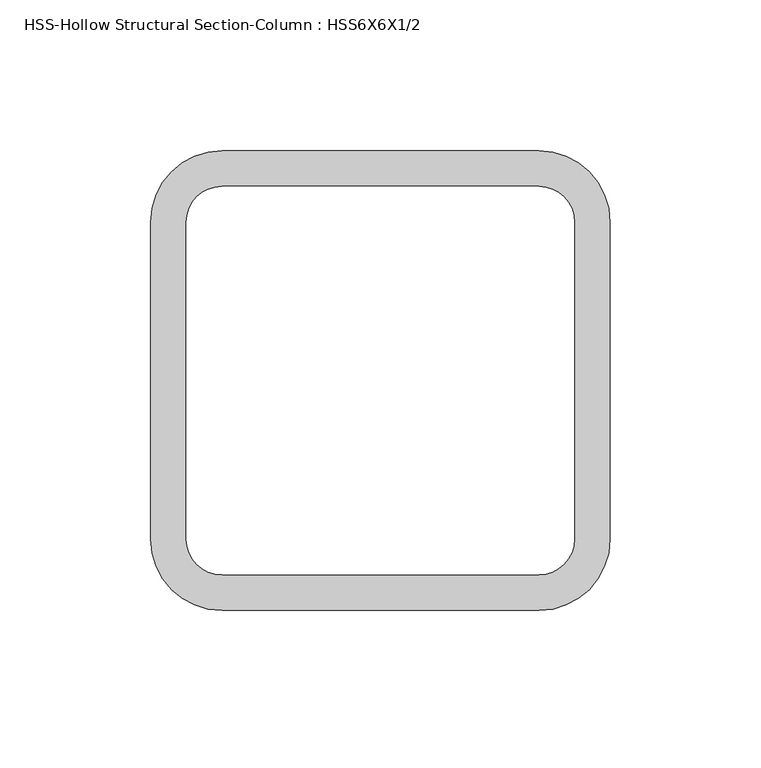
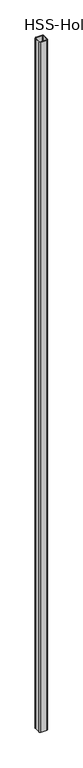
"""IFC4 building model written with IfcOpenShell, lengths in millimetres: column geometry, HSS-Hollow Structural Section-Column : HSS6X6X1/2."""

import ifcopenshell
import ifcopenshell.guid

model = None  # the IFC model being written
_history = None  # IfcOwnerHistory: only IFC2X3 demands one
_inside = {}  # id of a spatial element -> (the spatial element, [elements in it])
_under = {}  # id of a project, library or spatial element -> (it, [spatial elements below it])
_declared = {}  # id of a project -> (the project, [libraries it declares])
_typed = {}  # id of a type object -> (the type object, [elements of that type])
_made_of = {}  # id of a material, layer set ... -> (it, [elements and type objects made of it])


def new_model(schema):
    """Start an empty IFC model of exactly this schema.

    Asked for "IFC4X3", IfcOpenShell would pick the latest addendum, in which some entities
    have other attributes; the version numbers below select the first issue.
    IFC2X3 requires an IfcOwnerHistory on every rooted entity: one is made here for all.
    """
    global model, _history
    if schema == "IFC4X3":
        model = ifcopenshell.file(schema_version=(4, 3, 0, 0))
    else:
        model = ifcopenshell.file(schema=schema)
    _inside.clear()
    _under.clear()
    _declared.clear()
    _typed.clear()
    _made_of.clear()
    _history = None
    if model.schema == "IFC2X3":
        org = make("IfcOrganization", Name="unknown")
        user = make(
            "IfcPersonAndOrganization",
            ThePerson=make("IfcPerson", FamilyName="unknown"),
            TheOrganization=org,
        )
        app = make(
            "IfcApplication",
            ApplicationDeveloper=org,
            Version="unknown",
            ApplicationFullName="unknown",
            ApplicationIdentifier="unknown",
        )
        _history = make(
            "IfcOwnerHistory",
            OwningUser=user,
            OwningApplication=app,
            ChangeAction="ADDED",
            CreationDate=0,
        )
    return model


def make(cls, **values):
    """One entity of the class cls with the attributes given. An attribute that is None is left unset."""
    return model.create_entity(
        cls, **{name: value for name, value in values.items() if value is not None}
    )


def rooted(cls, **values):
    """An entity with a GlobalId (a new one), such as an element, a storey or a relation."""
    return make(cls, GlobalId=ifcopenshell.guid.new(), OwnerHistory=_history, **values)


def si_unit(unit_type, name, prefix=None):
    """IfcSIUnit, for example si_unit("LENGTHUNIT", "METRE", prefix="MILLI")."""
    return make("IfcSIUnit", UnitType=unit_type, Prefix=prefix, Name=name)


def assignment(units):
    """IfcUnitAssignment: the units of a project."""
    return None if units is None else make("IfcUnitAssignment", Units=units)


def point(xyz):
    """IfcCartesianPoint."""
    return None if xyz is None else make("IfcCartesianPoint", Coordinates=xyz)


def direction(xyz):
    """IfcDirection."""
    return None if xyz is None else make("IfcDirection", DirectionRatios=xyz)


def frame(location, z_axis=None, x_axis=None):
    """IfcAxis2Placement3D, a coordinate frame: its origin and axes. An axis left out is left unset."""
    return make(
        "IfcAxis2Placement3D",
        Location=point(location),
        Axis=direction(z_axis),
        RefDirection=direction(x_axis),
    )


def frame_2d(location, x_axis=None):
    """IfcAxis2Placement2D, a coordinate frame in the plane: its origin and x axis."""
    return make(
        "IfcAxis2Placement2D", Location=point(location), RefDirection=direction(x_axis)
    )


def origin():
    """The frame at (0, 0, 0) with its axes left unset."""
    return frame((0.0, 0.0, 0.0))


def place(relative_to, where):
    """IfcLocalPlacement: puts the frame where relative to a parent placement (None: the world)."""
    return make(
        "IfcLocalPlacement", PlacementRelTo=relative_to, RelativePlacement=where
    )


def context(
    kind, dimensions, precision=None, world=None, true_north=None, identifier=None
):
    """IfcGeometricRepresentationContext, for example the 3D "Model" context."""
    return make(
        "IfcGeometricRepresentationContext",
        ContextIdentifier=identifier,
        ContextType=kind,
        CoordinateSpaceDimension=dimensions,
        Precision=precision,
        WorldCoordinateSystem=world,
        TrueNorth=true_north,
    )


def project(units=None, contexts=None):
    """IfcProject with its units and contexts."""
    return rooted(
        "IfcProject",
        Name="project",
        RepresentationContexts=contexts,
        UnitsInContext=assignment(units),
    )


def spatial(cls, under=None, at=None, **own):
    """A site, building, storey or space (cls), placed at a placement, below another one or the project."""
    s = rooted(cls, ObjectPlacement=at, **own)
    if under is not None:
        _under.setdefault(under.id(), (under, []))[1].append(s)
    return s


def polyline(points):
    """IfcPolyline through the points."""
    return make("IfcPolyline", Points=[point(p) for p in points])


def circle_curve(where, radius):
    """IfcCircle in the frame where."""
    return make("IfcCircle", Position=where, Radius=radius)


def trimmed(basis, trim1, trim2, sense, master):
    """IfcTrimmedCurve: the piece of a basis curve between two trims."""
    return make(
        "IfcTrimmedCurve",
        BasisCurve=basis,
        Trim1=trim1,
        Trim2=trim2,
        SenseAgreement=sense,
        MasterRepresentation=master,
    )


def segment(curve, same_sense, transition):
    """IfcCompositeCurveSegment."""
    return make(
        "IfcCompositeCurveSegment",
        Transition=transition,
        SameSense=same_sense,
        ParentCurve=curve,
    )


def composite_curve(segments, self_intersect=None):
    """IfcCompositeCurve: segments joined end to end."""
    return make("IfcCompositeCurve", Segments=segments, SelfIntersect=self_intersect)


def outline(outer, holes=None, kind="AREA"):
    """IfcArbitraryClosedProfileDef: a profile drawn as a closed curve; with holes, ...WithVoids."""
    if holes is None:
        return make("IfcArbitraryClosedProfileDef", ProfileType=kind, OuterCurve=outer)
    return make(
        "IfcArbitraryProfileDefWithVoids",
        ProfileType=kind,
        OuterCurve=outer,
        InnerCurves=holes,
    )


def extrude(swept, where, along, depth):
    """IfcExtrudedAreaSolid: the profile swept, set in the frame where, extruded along a direction by depth."""
    return make(
        "IfcExtrudedAreaSolid",
        SweptArea=swept,
        Position=where,
        ExtrudedDirection=direction(along),
        Depth=depth,
    )


def shape(context_of_items, identifier, shape_type, items):
    """IfcShapeRepresentation: the items that make up one representation, for example the "Body"."""
    return make(
        "IfcShapeRepresentation",
        ContextOfItems=context_of_items,
        RepresentationIdentifier=identifier,
        RepresentationType=shape_type,
        Items=items,
    )


def source(mapping_origin, context_of_items, identifier, shape_type, items):
    """IfcRepresentationMap: a shape defined once, which mapped items show again and again."""
    return make(
        "IfcRepresentationMap",
        MappingOrigin=mapping_origin,
        MappedRepresentation=shape(context_of_items, identifier, shape_type, items),
    )


def transform(
    local_origin,
    x_axis=None,
    y_axis=None,
    z_axis=None,
    scale=None,
    scale2=None,
    scale3=None,
    uniform=True,
):
    """IfcCartesianTransformationOperator3D, or its non-uniform kind. x_axis, y_axis, z_axis: its Axis1, 2, 3."""
    if uniform:
        return make(
            "IfcCartesianTransformationOperator3D",
            Axis1=direction(x_axis),
            Axis2=direction(y_axis),
            LocalOrigin=point(local_origin),
            Scale=scale,
            Axis3=direction(z_axis),
        )
    return make(
        "IfcCartesianTransformationOperator3DnonUniform",
        Axis1=direction(x_axis),
        Axis2=direction(y_axis),
        LocalOrigin=point(local_origin),
        Scale=scale,
        Axis3=direction(z_axis),
        Scale2=scale2,
        Scale3=scale3,
    )


def mapped(mapping_source, mapping_target):
    """IfcMappedItem: shows the shape of a source again, moved by a transform."""
    return make(
        "IfcMappedItem", MappingSource=mapping_source, MappingTarget=mapping_target
    )


def made_of(thing, what):
    """Note that an element or type object is made of a material, layer set ...; save() writes the relation."""
    if what is not None:
        _made_of.setdefault(what.id(), (what, []))[1].append(thing)
    return thing


def element(
    cls,
    number,
    at=None,
    inside=None,
    cuts=None,
    type_object=None,
    material=None,
    context=None,
    identifier="Body",
    shape_type=None,
    held_by="IfcProductDefinitionShape",
    body=None,
    shapes=None,
    **own,
):
    """One element of the class cls, such as IfcWall. Its Tag is "e" and its number.

    at: its placement. inside: the storey or other place that contains it. cuts: it is an
    opening in that element (IfcRelVoidsElement). A single representation is given by context,
    identifier, shape_type and body (its items); several are given by shapes. held_by: the class
    of the entity that holds the representations. save() writes the other relations.
    """
    e = rooted(cls, Tag="e%d" % number, ObjectPlacement=at, **own)
    if body is not None:
        shapes = [shape(context, identifier, shape_type, body)]
    if shapes is not None:
        e.Representation = make(held_by, Representations=shapes)
    if inside is not None:
        _inside.setdefault(inside.id(), (inside, []))[1].append(e)
    if cuts is not None:
        rooted(
            "IfcRelVoidsElement", RelatingBuildingElement=cuts, RelatedOpeningElement=e
        )
    if type_object is not None:
        _typed.setdefault(type_object.id(), (type_object, []))[1].append(e)
    return made_of(e, material)


def aggregate(whole, parts):
    """IfcRelAggregates: a whole, such as a stair, and the parts it consists of."""
    return rooted("IfcRelAggregates", RelatingObject=whole, RelatedObjects=parts)


def save(model, path):
    """Write the relations noted so far, then the file.

    IfcRelAggregates (storeys below a building ...), IfcRelContainedInSpatialStructure (elements
    in a storey), IfcRelDefinesByType, IfcRelAssociatesMaterial and IfcRelDeclares: one each for
    every whole, place, type object, material and project.
    """
    for whole, parts in _under.values():
        aggregate(whole, parts)
    for where, things in _inside.values():
        rooted(
            "IfcRelContainedInSpatialStructure",
            RelatedElements=things,
            RelatingStructure=where,
        )
    for kind, things in _typed.values():
        rooted("IfcRelDefinesByType", RelatedObjects=things, RelatingType=kind)
    for what, things in _made_of.values():
        rooted("IfcRelAssociatesMaterial", RelatedObjects=things, RelatingMaterial=what)
    for by, libraries in _declared.values():
        rooted("IfcRelDeclares", RelatingContext=by, RelatedDefinitions=libraries)
    model.write(path)


def hss_hollow_structural_section_column_hss6x6x1_2_509d929d(model_context):
    return source(origin(), model_context, "Body", "SweptSolid", [
        extrude(outline(composite_curve([segment(trimmed(circle_curve(frame_2d((52.578, 52.578)), 23.622), [point((52.578, 76.2))], [point((76.2, 52.578))], False, "CARTESIAN"), True, "CONTINUOUS"), segment(polyline([(76.2, 52.578), (76.2, -52.578)]), True, "CONTINUOUS"), segment(trimmed(circle_curve(frame_2d((52.578, -52.578)), 23.622), [point((76.2, -52.578))], [point((52.578, -76.2))], False, "CARTESIAN"), True, "CONTINUOUS"), segment(polyline([(52.578, -76.2), (-52.578, -76.2)]), True, "CONTINUOUS"), segment(trimmed(circle_curve(frame_2d((-52.578, -52.578)), 23.622), [point((-52.578, -76.2))], [point((-76.2, -52.578))], False, "CARTESIAN"), True, "CONTINUOUS"), segment(polyline([(-76.2, -52.578), (-76.2, 52.578)]), True, "CONTINUOUS"), segment(trimmed(circle_curve(frame_2d((-52.578, 52.578)), 23.622), [point((-76.2, 52.578))], [point((-52.578, 76.2))], False, "CARTESIAN"), True, "CONTINUOUS"), segment(polyline([(-52.578, 76.2), (52.578, 76.2)]), True, "CONTINUOUS")], self_intersect=False), holes=[composite_curve([segment(polyline([(52.578, 64.389), (-52.578, 64.389)]), True, "CONTINUOUS"), segment(trimmed(circle_curve(frame_2d((-52.578, 52.578)), 11.811), [point((-52.578, 64.389))], [point((-64.389, 52.578))], True, "CARTESIAN"), True, "CONTINUOUS"), segment(polyline([(-64.389, 52.578), (-64.389, -52.578)]), True, "CONTINUOUS"), segment(trimmed(circle_curve(frame_2d((-52.578, -52.578)), 11.811), [point((-64.389, -52.578))], [point((-52.578, -64.389))], True, "CARTESIAN"), True, "CONTINUOUS"), segment(polyline([(-52.578, -64.389), (52.578, -64.389)]), True, "CONTINUOUS"), segment(trimmed(circle_curve(frame_2d((52.578, -52.578)), 11.811), [point((52.578, -64.389))], [point((64.389, -52.578))], True, "CARTESIAN"), True, "CONTINUOUS"), segment(polyline([(64.389, -52.578), (64.389, 52.578)]), True, "CONTINUOUS"), segment(trimmed(circle_curve(frame_2d((52.578, 52.578)), 11.811), [point((64.389, 52.578))], [point((52.578, 64.389))], True, "CARTESIAN"), True, "CONTINUOUS")], self_intersect=False)]), frame((0.0, 0.0, -609.6), z_axis=(0.0, 0.0, 1.0), x_axis=(1.0, 0.0, 0.0)), (0.0, 0.0, 1.0), 13004.8),
    ])


if __name__ == "__main__":
    model = new_model("IFC4")
    model_context = context("Model", 3, world=origin())
    ifc_project = project(units=[si_unit("LENGTHUNIT", "METRE", prefix="MILLI")], contexts=[model_context])
    site = spatial("IfcSite", under=ifc_project)
    building = spatial("IfcBuilding", under=site)
    placement = place(None, origin())
    hss_hollow_structural_section_column_hss6x6x1_2_shape = hss_hollow_structural_section_column_hss6x6x1_2_509d929d(model_context)
    element("IfcColumn", 1, ObjectType="HSS-Hollow Structural Section-Column : HSS6X6X1/2", at=placement, inside=building, context=model_context, shape_type="MappedRepresentation", body=[
        mapped(hss_hollow_structural_section_column_hss6x6x1_2_shape, transform((0.0, 0.0, 0.0), x_axis=(1.0, 0.0, 0.0), y_axis=(0.0, 1.0, 0.0), z_axis=(0.0, 0.0, 1.0))),
    ])
    save(model, "model.ifc")

# Revit data of these elements
# Type "HSS-Hollow Structural Section-Column : HSS6X6X1/2"
#   Assembly Code = "B10"
#   Shape = "Square"
#   W = 35.1
#   Ht = 0' - 6"
#   b = 0' - 6"
#   kr = 0' - 0.93"
#   t = 0' - 0.465"
#   A = 0.0676389 SF
#   Structural Material [instance default] = Steel ASTM A500, Grade B, Rectangular and Square
# Element 1 (IfcColumn, "HSS-Hollow Structural Section-Column : HSS6X6X1/2")
#   Materials on its faces: "Steel ASTM A500, Grade B, Rectangular and Square"
# Materials
#   "Steel ASTM A500, Grade B, Rectangular and Square": class "Metal", colour RGB 199 199 199, transparency 0, Description = "Carbon steel", Cost = 0
